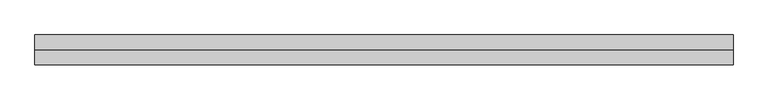
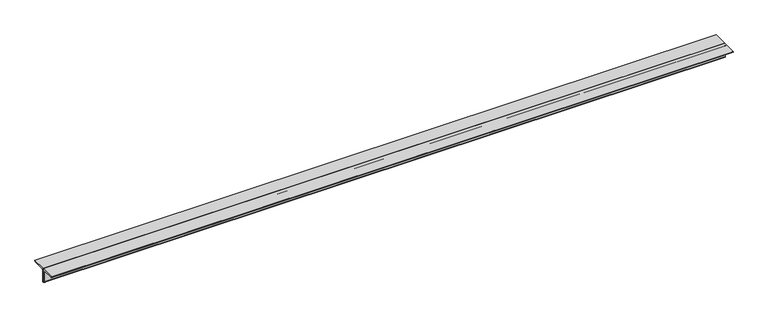
"""IFC4 building model written with IfcOpenShell, lengths in millimetres: member geometry, 0123_Steel Framing_2Ls-KSD3502 : H_SB_AR_S04_2Ls-130x130x12_VBR2."""

from ifc_helpers import new_model, si_unit, point, frame, frame_2d, origin, place, context, project, spatial, polyline, circle_curve, trimmed, segment, composite_curve, outline, extrude, source, transform, mapped, element, save


def member_a61622f5(model_context):
    return source(origin(), model_context, "Body", "SweptSolid", [
        extrude(outline(composite_curve([segment(polyline([(0.0, 36.4), (130.0, 36.4)]), True, "CONTINUOUS"), segment(trimmed(circle_curve(frame_2d((118.0, 36.4)), 12.0), [point((130.0, 36.4))], [point((118.0, 24.4))], False, "CARTESIAN"), True, "CONTINUOUS"), segment(polyline([(118.0, 24.4), (24.0, 24.4)]), True, "CONTINUOUS"), segment(trimmed(circle_curve(frame_2d((24.0, 12.4)), 12.0), [point((24.0, 24.4))], [point((12.0, 12.4))], True, "CARTESIAN"), True, "CONTINUOUS"), segment(polyline([(12.0, 12.4), (12.0, -81.6)]), True, "CONTINUOUS"), segment(trimmed(circle_curve(frame_2d((0.0, -81.6)), 12.0), [point((12.0, -81.6))], [point((0.0, -93.6))], False, "CARTESIAN"), True, "CONTINUOUS"), segment(polyline([(0.0, -93.6), (0.0, 36.4)]), True, "CONTINUOUS")], self_intersect=False)), frame((-3093.2366876, 0.0, 0.0), z_axis=(1.0, 0.0, 0.0), x_axis=(0.0, 1.0, 0.0)), (0.0, 0.0, 1.0), 6055.217292),
        extrude(outline(composite_curve([segment(polyline([(0.0, 36.4), (0.0, -93.6)]), True, "CONTINUOUS"), segment(trimmed(circle_curve(frame_2d((0.0, -81.6)), 12.0), [point((0.0, -93.6))], [point((-12.0, -81.6))], False, "CARTESIAN"), True, "CONTINUOUS"), segment(polyline([(-12.0, -81.6), (-12.0, 12.4)]), True, "CONTINUOUS"), segment(trimmed(circle_curve(frame_2d((-24.0, 12.4)), 12.0), [point((-12.0, 12.4))], [point((-24.0, 24.4))], True, "CARTESIAN"), True, "CONTINUOUS"), segment(polyline([(-24.0, 24.4), (-118.0, 24.4)]), True, "CONTINUOUS"), segment(trimmed(circle_curve(frame_2d((-118.0, 36.4)), 12.0), [point((-118.0, 24.4))], [point((-130.0, 36.4))], False, "CARTESIAN"), True, "CONTINUOUS"), segment(polyline([(-130.0, 36.4), (0.0, 36.4)]), True, "CONTINUOUS")], self_intersect=False)), frame((-3093.2366876, 0.0, 0.0), z_axis=(1.0, 0.0, 0.0), x_axis=(0.0, 1.0, 0.0)), (0.0, 0.0, 1.0), 6055.217292),
    ])


if __name__ == "__main__":
    model = new_model("IFC4")
    model_context = context("Model", 3, world=origin())
    ifc_project = project(units=[si_unit("LENGTHUNIT", "METRE", prefix="MILLI")], contexts=[model_context])
    site = spatial("IfcSite", under=ifc_project)
    building = spatial("IfcBuilding", under=site)
    placement = place(None, origin())
    member_shape = member_a61622f5(model_context)
    element("IfcMember", 1, ObjectType="0123_Steel Framing_2Ls-KSD3502 : H_SB_AR_S04_2Ls-130x130x12_VBR2", at=placement, inside=building, context=model_context, shape_type="MappedRepresentation", body=[
        mapped(member_shape, transform((0.0, 0.0, 0.0), x_axis=(1.0, 0.0, 0.0), y_axis=(0.0, 1.0, 0.0), z_axis=(0.0, 0.0, 1.0))),
    ])
    save(model, "model.ifc")

# Revit data of these elements
# Type "0123_Steel Framing_2Ls-KSD3502 : H_SB_AR_S04_2Ls-130x130x12_VBR2"
#   Assembly Code = "B10"
#   Legs = "SLBB"
#   W = 8.97
#   Perimeter = 1.04 m²/m
#   Nominal Weight = 46.80 kgf/m
#   Length [instance default] = 1000 mm
#   Space = 0 mm
#   b = 130 mm
#   d = 130 mm
#   t = 12 mm
#   y = 36.4 mm
#   A = 0.005952 m²
#   Structural Material [instance default] = Steel ASTM A36
# Element 1 (IfcMember, "0123_Steel Framing_2Ls-KSD3502 : H_SB_AR_S04_2Ls-130x130x12_VBR2")
#   Structural Material = Steel, 45-345
#   Materials on its faces: "Steel, 45-345"
# Materials
#   "Steel ASTM A36": class "Metal", colour RGB 199 199 199, transparency 0, Description = "Structural steel, ASTM A36 Grade B, mill finish", Cost = 0
#   "Steel, 45-345": class "Metal", colour RGB 189 187 185, transparency 0, Description = "Steel 345 MPa", Cost = 0
